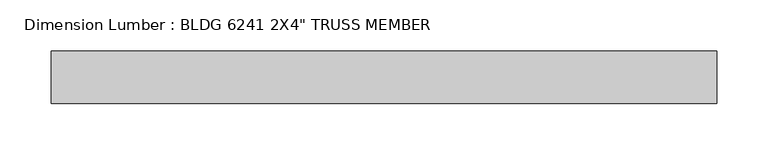
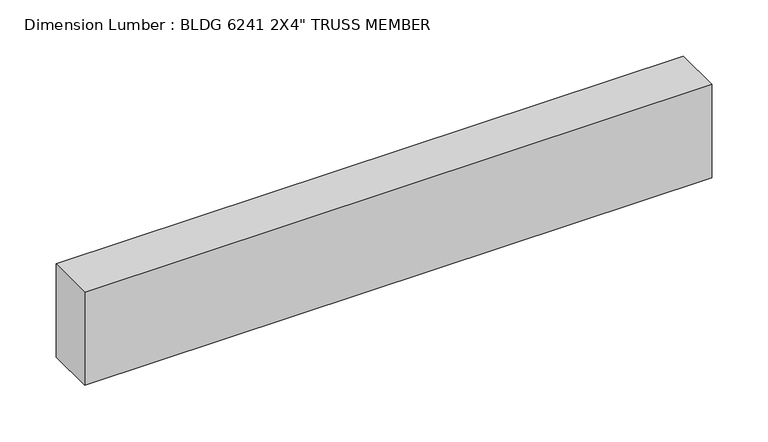
"""IFC4 building model written with IfcOpenShell, lengths in millimetres: beam geometry."""

import ifcopenshell
import ifcopenshell.guid

model = None  # the IFC model being written
_history = None  # IfcOwnerHistory: only IFC2X3 demands one
_inside = {}  # id of a spatial element -> (the spatial element, [elements in it])
_under = {}  # id of a project, library or spatial element -> (it, [spatial elements below it])
_declared = {}  # id of a project -> (the project, [libraries it declares])
_typed = {}  # id of a type object -> (the type object, [elements of that type])
_made_of = {}  # id of a material, layer set ... -> (it, [elements and type objects made of it])


def new_model(schema):
    """Start an empty IFC model of exactly this schema.

    Asked for "IFC4X3", IfcOpenShell would pick the latest addendum, in which some entities
    have other attributes; the version numbers below select the first issue.
    IFC2X3 requires an IfcOwnerHistory on every rooted entity: one is made here for all.
    """
    global model, _history
    if schema == "IFC4X3":
        model = ifcopenshell.file(schema_version=(4, 3, 0, 0))
    else:
        model = ifcopenshell.file(schema=schema)
    _inside.clear()
    _under.clear()
    _declared.clear()
    _typed.clear()
    _made_of.clear()
    _history = None
    if model.schema == "IFC2X3":
        org = make("IfcOrganization", Name="unknown")
        user = make(
            "IfcPersonAndOrganization",
            ThePerson=make("IfcPerson", FamilyName="unknown"),
            TheOrganization=org,
        )
        app = make(
            "IfcApplication",
            ApplicationDeveloper=org,
            Version="unknown",
            ApplicationFullName="unknown",
            ApplicationIdentifier="unknown",
        )
        _history = make(
            "IfcOwnerHistory",
            OwningUser=user,
            OwningApplication=app,
            ChangeAction="ADDED",
            CreationDate=0,
        )
    return model


def make(cls, **values):
    """One entity of the class cls with the attributes given. An attribute that is None is left unset."""
    return model.create_entity(
        cls, **{name: value for name, value in values.items() if value is not None}
    )


def rooted(cls, **values):
    """An entity with a GlobalId (a new one), such as an element, a storey or a relation."""
    return make(cls, GlobalId=ifcopenshell.guid.new(), OwnerHistory=_history, **values)


def si_unit(unit_type, name, prefix=None):
    """IfcSIUnit, for example si_unit("LENGTHUNIT", "METRE", prefix="MILLI")."""
    return make("IfcSIUnit", UnitType=unit_type, Prefix=prefix, Name=name)


def assignment(units):
    """IfcUnitAssignment: the units of a project."""
    return None if units is None else make("IfcUnitAssignment", Units=units)


def point(xyz):
    """IfcCartesianPoint."""
    return None if xyz is None else make("IfcCartesianPoint", Coordinates=xyz)


def direction(xyz):
    """IfcDirection."""
    return None if xyz is None else make("IfcDirection", DirectionRatios=xyz)


def frame(location, z_axis=None, x_axis=None):
    """IfcAxis2Placement3D, a coordinate frame: its origin and axes. An axis left out is left unset."""
    return make(
        "IfcAxis2Placement3D",
        Location=point(location),
        Axis=direction(z_axis),
        RefDirection=direction(x_axis),
    )


def origin():
    """The frame at (0, 0, 0) with its axes left unset."""
    return frame((0.0, 0.0, 0.0))


def place(relative_to, where):
    """IfcLocalPlacement: puts the frame where relative to a parent placement (None: the world)."""
    return make(
        "IfcLocalPlacement", PlacementRelTo=relative_to, RelativePlacement=where
    )


def context(
    kind, dimensions, precision=None, world=None, true_north=None, identifier=None
):
    """IfcGeometricRepresentationContext, for example the 3D "Model" context."""
    return make(
        "IfcGeometricRepresentationContext",
        ContextIdentifier=identifier,
        ContextType=kind,
        CoordinateSpaceDimension=dimensions,
        Precision=precision,
        WorldCoordinateSystem=world,
        TrueNorth=true_north,
    )


def project(units=None, contexts=None):
    """IfcProject with its units and contexts."""
    return rooted(
        "IfcProject",
        Name="project",
        RepresentationContexts=contexts,
        UnitsInContext=assignment(units),
    )


def spatial(cls, under=None, at=None, **own):
    """A site, building, storey or space (cls), placed at a placement, below another one or the project."""
    s = rooted(cls, ObjectPlacement=at, **own)
    if under is not None:
        _under.setdefault(under.id(), (under, []))[1].append(s)
    return s


def polyline(points):
    """IfcPolyline through the points."""
    return make("IfcPolyline", Points=[point(p) for p in points])


def outline(outer, holes=None, kind="AREA"):
    """IfcArbitraryClosedProfileDef: a profile drawn as a closed curve; with holes, ...WithVoids."""
    if holes is None:
        return make("IfcArbitraryClosedProfileDef", ProfileType=kind, OuterCurve=outer)
    return make(
        "IfcArbitraryProfileDefWithVoids",
        ProfileType=kind,
        OuterCurve=outer,
        InnerCurves=holes,
    )


def extrude(swept, where, along, depth):
    """IfcExtrudedAreaSolid: the profile swept, set in the frame where, extruded along a direction by depth."""
    return make(
        "IfcExtrudedAreaSolid",
        SweptArea=swept,
        Position=where,
        ExtrudedDirection=direction(along),
        Depth=depth,
    )


def shape(context_of_items, identifier, shape_type, items):
    """IfcShapeRepresentation: the items that make up one representation, for example the "Body"."""
    return make(
        "IfcShapeRepresentation",
        ContextOfItems=context_of_items,
        RepresentationIdentifier=identifier,
        RepresentationType=shape_type,
        Items=items,
    )


def source(mapping_origin, context_of_items, identifier, shape_type, items):
    """IfcRepresentationMap: a shape defined once, which mapped items show again and again."""
    return make(
        "IfcRepresentationMap",
        MappingOrigin=mapping_origin,
        MappedRepresentation=shape(context_of_items, identifier, shape_type, items),
    )


def transform(
    local_origin,
    x_axis=None,
    y_axis=None,
    z_axis=None,
    scale=None,
    scale2=None,
    scale3=None,
    uniform=True,
):
    """IfcCartesianTransformationOperator3D, or its non-uniform kind. x_axis, y_axis, z_axis: its Axis1, 2, 3."""
    if uniform:
        return make(
            "IfcCartesianTransformationOperator3D",
            Axis1=direction(x_axis),
            Axis2=direction(y_axis),
            LocalOrigin=point(local_origin),
            Scale=scale,
            Axis3=direction(z_axis),
        )
    return make(
        "IfcCartesianTransformationOperator3DnonUniform",
        Axis1=direction(x_axis),
        Axis2=direction(y_axis),
        LocalOrigin=point(local_origin),
        Scale=scale,
        Axis3=direction(z_axis),
        Scale2=scale2,
        Scale3=scale3,
    )


def mapped(mapping_source, mapping_target):
    """IfcMappedItem: shows the shape of a source again, moved by a transform."""
    return make(
        "IfcMappedItem", MappingSource=mapping_source, MappingTarget=mapping_target
    )


def made_of(thing, what):
    """Note that an element or type object is made of a material, layer set ...; save() writes the relation."""
    if what is not None:
        _made_of.setdefault(what.id(), (what, []))[1].append(thing)
    return thing


def element(
    cls,
    number,
    at=None,
    inside=None,
    cuts=None,
    type_object=None,
    material=None,
    context=None,
    identifier="Body",
    shape_type=None,
    held_by="IfcProductDefinitionShape",
    body=None,
    shapes=None,
    **own,
):
    """One element of the class cls, such as IfcWall. Its Tag is "e" and its number.

    at: its placement. inside: the storey or other place that contains it. cuts: it is an
    opening in that element (IfcRelVoidsElement). A single representation is given by context,
    identifier, shape_type and body (its items); several are given by shapes. held_by: the class
    of the entity that holds the representations. save() writes the other relations.
    """
    e = rooted(cls, Tag="e%d" % number, ObjectPlacement=at, **own)
    if body is not None:
        shapes = [shape(context, identifier, shape_type, body)]
    if shapes is not None:
        e.Representation = make(held_by, Representations=shapes)
    if inside is not None:
        _inside.setdefault(inside.id(), (inside, []))[1].append(e)
    if cuts is not None:
        rooted(
            "IfcRelVoidsElement", RelatingBuildingElement=cuts, RelatedOpeningElement=e
        )
    if type_object is not None:
        _typed.setdefault(type_object.id(), (type_object, []))[1].append(e)
    return made_of(e, material)


def aggregate(whole, parts):
    """IfcRelAggregates: a whole, such as a stair, and the parts it consists of."""
    return rooted("IfcRelAggregates", RelatingObject=whole, RelatedObjects=parts)


def save(model, path):
    """Write the relations noted so far, then the file.

    IfcRelAggregates (storeys below a building ...), IfcRelContainedInSpatialStructure (elements
    in a storey), IfcRelDefinesByType, IfcRelAssociatesMaterial and IfcRelDeclares: one each for
    every whole, place, type object, material and project.
    """
    for whole, parts in _under.values():
        aggregate(whole, parts)
    for where, things in _inside.values():
        rooted(
            "IfcRelContainedInSpatialStructure",
            RelatedElements=things,
            RelatingStructure=where,
        )
    for kind, things in _typed.values():
        rooted("IfcRelDefinesByType", RelatedObjects=things, RelatingType=kind)
    for what, things in _made_of.values():
        rooted("IfcRelAssociatesMaterial", RelatedObjects=things, RelatingMaterial=what)
    for by, libraries in _declared.values():
        rooted("IfcRelDeclares", RelatingContext=by, RelatedDefinitions=libraries)
    model.write(path)


def beam_99e5442a(model_context):
    return source(origin(), model_context, "Body", "SweptSolid", [
        extrude(outline(polyline([(350.5042173, -25.4), (-295.4519367, -25.4), (-295.4519367, 25.4), (350.5042173, 25.4), (350.5042173, -25.4)])), frame((0.0, 0.0, -50.8), z_axis=(0.0, 0.0, 1.0), x_axis=(1.0, 0.0, 0.0)), (0.0, 0.0, 1.0), 101.6),
    ])


if __name__ == "__main__":
    model = new_model("IFC4")
    model_context = context("Model", 3, world=origin())
    ifc_project = project(units=[si_unit("LENGTHUNIT", "METRE", prefix="MILLI")], contexts=[model_context])
    site = spatial("IfcSite", under=ifc_project)
    building = spatial("IfcBuilding", under=site)
    placement = place(None, origin())
    beam_shape = beam_99e5442a(model_context)
    element("IfcBeam", 1, ObjectType="Dimension Lumber : BLDG 6241 2X4\" TRUSS MEMBER", at=placement, inside=building, context=model_context, shape_type="MappedRepresentation", body=[
        mapped(beam_shape, transform((0.0, 0.0, 0.0), x_axis=(1.0, 0.0, 0.0), y_axis=(0.0, 1.0, 0.0), z_axis=(0.0, 0.0, 1.0))),
    ])
    save(model, "model.ifc")

# Revit data of these elements
# Type "Dimension Lumber : BLDG 6241 2X4\" TRUSS MEMBER"
#   Assembly Code = "B10"
#   A = 0.273472 SF
#   Length [instance default] = 5' - 0"
#   b = 0' - 2"
#   d = 0' - 4"
#   Structural Material [instance default] = Softwood, Lumber
# Element 1 (IfcBeam, "Dimension Lumber : BLDG 6241 2X4\" TRUSS MEMBER")
#   Materials on its faces: "Softwood, Lumber"
# Materials
#   "Softwood, Lumber": class "Wood", colour RGB 223 192 134, transparency 0, Description = "Pinus Echinata", Cost = 0
